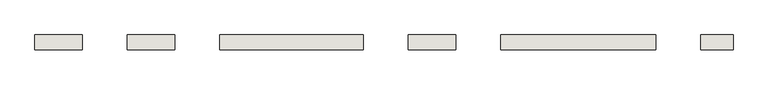
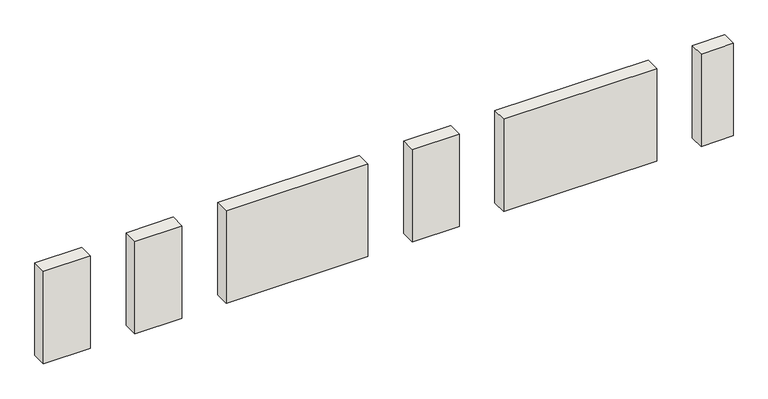
"""IFC4 building model written with IfcOpenShell, lengths in millimetres: wall geometry, 0_3d."""

import ifcopenshell
import ifcopenshell.guid

model = None  # the IFC model being written
_history = None  # IfcOwnerHistory: only IFC2X3 demands one
_inside = {}  # id of a spatial element -> (the spatial element, [elements in it])
_under = {}  # id of a project, library or spatial element -> (it, [spatial elements below it])
_declared = {}  # id of a project -> (the project, [libraries it declares])
_typed = {}  # id of a type object -> (the type object, [elements of that type])
_made_of = {}  # id of a material, layer set ... -> (it, [elements and type objects made of it])


def new_model(schema):
    """Start an empty IFC model of exactly this schema.

    Asked for "IFC4X3", IfcOpenShell would pick the latest addendum, in which some entities
    have other attributes; the version numbers below select the first issue.
    IFC2X3 requires an IfcOwnerHistory on every rooted entity: one is made here for all.
    """
    global model, _history
    if schema == "IFC4X3":
        model = ifcopenshell.file(schema_version=(4, 3, 0, 0))
    else:
        model = ifcopenshell.file(schema=schema)
    _inside.clear()
    _under.clear()
    _declared.clear()
    _typed.clear()
    _made_of.clear()
    _history = None
    if model.schema == "IFC2X3":
        org = make("IfcOrganization", Name="unknown")
        user = make(
            "IfcPersonAndOrganization",
            ThePerson=make("IfcPerson", FamilyName="unknown"),
            TheOrganization=org,
        )
        app = make(
            "IfcApplication",
            ApplicationDeveloper=org,
            Version="unknown",
            ApplicationFullName="unknown",
            ApplicationIdentifier="unknown",
        )
        _history = make(
            "IfcOwnerHistory",
            OwningUser=user,
            OwningApplication=app,
            ChangeAction="ADDED",
            CreationDate=0,
        )
    return model


def make(cls, **values):
    """One entity of the class cls with the attributes given. An attribute that is None is left unset."""
    return model.create_entity(
        cls, **{name: value for name, value in values.items() if value is not None}
    )


def rooted(cls, **values):
    """An entity with a GlobalId (a new one), such as an element, a storey or a relation."""
    return make(cls, GlobalId=ifcopenshell.guid.new(), OwnerHistory=_history, **values)


def si_unit(unit_type, name, prefix=None):
    """IfcSIUnit, for example si_unit("LENGTHUNIT", "METRE", prefix="MILLI")."""
    return make("IfcSIUnit", UnitType=unit_type, Prefix=prefix, Name=name)


def assignment(units):
    """IfcUnitAssignment: the units of a project."""
    return None if units is None else make("IfcUnitAssignment", Units=units)


def point(xyz):
    """IfcCartesianPoint."""
    return None if xyz is None else make("IfcCartesianPoint", Coordinates=xyz)


def direction(xyz):
    """IfcDirection."""
    return None if xyz is None else make("IfcDirection", DirectionRatios=xyz)


def frame(location, z_axis=None, x_axis=None):
    """IfcAxis2Placement3D, a coordinate frame: its origin and axes. An axis left out is left unset."""
    return make(
        "IfcAxis2Placement3D",
        Location=point(location),
        Axis=direction(z_axis),
        RefDirection=direction(x_axis),
    )


def origin():
    """The frame at (0, 0, 0) with its axes left unset."""
    return frame((0.0, 0.0, 0.0))


def origin_with_axes():
    """The frame at (0, 0, 0) with the z axis (0, 0, 1) and the x axis (1, 0, 0) written out."""
    return frame((0.0, 0.0, 0.0), z_axis=(0.0, 0.0, 1.0), x_axis=(1.0, 0.0, 0.0))


def place(relative_to, where):
    """IfcLocalPlacement: puts the frame where relative to a parent placement (None: the world)."""
    return make(
        "IfcLocalPlacement", PlacementRelTo=relative_to, RelativePlacement=where
    )


def context(
    kind, dimensions, precision=None, world=None, true_north=None, identifier=None
):
    """IfcGeometricRepresentationContext, for example the 3D "Model" context."""
    return make(
        "IfcGeometricRepresentationContext",
        ContextIdentifier=identifier,
        ContextType=kind,
        CoordinateSpaceDimension=dimensions,
        Precision=precision,
        WorldCoordinateSystem=world,
        TrueNorth=true_north,
    )


def project(units=None, contexts=None):
    """IfcProject with its units and contexts."""
    return rooted(
        "IfcProject",
        Name="project",
        RepresentationContexts=contexts,
        UnitsInContext=assignment(units),
    )


def spatial(cls, under=None, at=None, **own):
    """A site, building, storey or space (cls), placed at a placement, below another one or the project."""
    s = rooted(cls, ObjectPlacement=at, **own)
    if under is not None:
        _under.setdefault(under.id(), (under, []))[1].append(s)
    return s


def polyline(points):
    """IfcPolyline through the points."""
    return make("IfcPolyline", Points=[point(p) for p in points])


def outline(outer, holes=None, kind="AREA"):
    """IfcArbitraryClosedProfileDef: a profile drawn as a closed curve; with holes, ...WithVoids."""
    if holes is None:
        return make("IfcArbitraryClosedProfileDef", ProfileType=kind, OuterCurve=outer)
    return make(
        "IfcArbitraryProfileDefWithVoids",
        ProfileType=kind,
        OuterCurve=outer,
        InnerCurves=holes,
    )


def extrude(swept, where, along, depth):
    """IfcExtrudedAreaSolid: the profile swept, set in the frame where, extruded along a direction by depth."""
    return make(
        "IfcExtrudedAreaSolid",
        SweptArea=swept,
        Position=where,
        ExtrudedDirection=direction(along),
        Depth=depth,
    )


def shape(context_of_items, identifier, shape_type, items):
    """IfcShapeRepresentation: the items that make up one representation, for example the "Body"."""
    return make(
        "IfcShapeRepresentation",
        ContextOfItems=context_of_items,
        RepresentationIdentifier=identifier,
        RepresentationType=shape_type,
        Items=items,
    )


def source(mapping_origin, context_of_items, identifier, shape_type, items):
    """IfcRepresentationMap: a shape defined once, which mapped items show again and again."""
    return make(
        "IfcRepresentationMap",
        MappingOrigin=mapping_origin,
        MappedRepresentation=shape(context_of_items, identifier, shape_type, items),
    )


def transform(
    local_origin,
    x_axis=None,
    y_axis=None,
    z_axis=None,
    scale=None,
    scale2=None,
    scale3=None,
    uniform=True,
):
    """IfcCartesianTransformationOperator3D, or its non-uniform kind. x_axis, y_axis, z_axis: its Axis1, 2, 3."""
    if uniform:
        return make(
            "IfcCartesianTransformationOperator3D",
            Axis1=direction(x_axis),
            Axis2=direction(y_axis),
            LocalOrigin=point(local_origin),
            Scale=scale,
            Axis3=direction(z_axis),
        )
    return make(
        "IfcCartesianTransformationOperator3DnonUniform",
        Axis1=direction(x_axis),
        Axis2=direction(y_axis),
        LocalOrigin=point(local_origin),
        Scale=scale,
        Axis3=direction(z_axis),
        Scale2=scale2,
        Scale3=scale3,
    )


def mapped(mapping_source, mapping_target):
    """IfcMappedItem: shows the shape of a source again, moved by a transform."""
    return make(
        "IfcMappedItem", MappingSource=mapping_source, MappingTarget=mapping_target
    )


def made_of(thing, what):
    """Note that an element or type object is made of a material, layer set ...; save() writes the relation."""
    if what is not None:
        _made_of.setdefault(what.id(), (what, []))[1].append(thing)
    return thing


def element(
    cls,
    number,
    at=None,
    inside=None,
    cuts=None,
    type_object=None,
    material=None,
    context=None,
    identifier="Body",
    shape_type=None,
    held_by="IfcProductDefinitionShape",
    body=None,
    shapes=None,
    **own,
):
    """One element of the class cls, such as IfcWall. Its Tag is "e" and its number.

    at: its placement. inside: the storey or other place that contains it. cuts: it is an
    opening in that element (IfcRelVoidsElement). A single representation is given by context,
    identifier, shape_type and body (its items); several are given by shapes. held_by: the class
    of the entity that holds the representations. save() writes the other relations.
    """
    e = rooted(cls, Tag="e%d" % number, ObjectPlacement=at, **own)
    if body is not None:
        shapes = [shape(context, identifier, shape_type, body)]
    if shapes is not None:
        e.Representation = make(held_by, Representations=shapes)
    if inside is not None:
        _inside.setdefault(inside.id(), (inside, []))[1].append(e)
    if cuts is not None:
        rooted(
            "IfcRelVoidsElement", RelatingBuildingElement=cuts, RelatedOpeningElement=e
        )
    if type_object is not None:
        _typed.setdefault(type_object.id(), (type_object, []))[1].append(e)
    return made_of(e, material)


def aggregate(whole, parts):
    """IfcRelAggregates: a whole, such as a stair, and the parts it consists of."""
    return rooted("IfcRelAggregates", RelatingObject=whole, RelatedObjects=parts)


def save(model, path):
    """Write the relations noted so far, then the file.

    IfcRelAggregates (storeys below a building ...), IfcRelContainedInSpatialStructure (elements
    in a storey), IfcRelDefinesByType, IfcRelAssociatesMaterial and IfcRelDeclares: one each for
    every whole, place, type object, material and project.
    """
    for whole, parts in _under.values():
        aggregate(whole, parts)
    for where, things in _inside.values():
        rooted(
            "IfcRelContainedInSpatialStructure",
            RelatedElements=things,
            RelatingStructure=where,
        )
    for kind, things in _typed.values():
        rooted("IfcRelDefinesByType", RelatedObjects=things, RelatingType=kind)
    for what, things in _made_of.values():
        rooted("IfcRelAssociatesMaterial", RelatedObjects=things, RelatingMaterial=what)
    for by, libraries in _declared.values():
        rooted("IfcRelDeclares", RelatingContext=by, RelatedDefinitions=libraries)
    model.write(path)


def wall_31735f31(model_context):
    return source(origin(), model_context, "Body", "SweptSolid", [
        extrude(outline(polyline([(1200.0, 380.0), (1200.0, 0.0), (0.0, 0.0), (0.0, 380.0), (1200.0, 380.0)])), origin_with_axes(), (0.0, 0.0, 1.0), 2500.0),
        extrude(outline(polyline([(2335.0, 0.0), (2335.0, 380.0), (3533.0664986, 380.0), (3533.0664986, 0.0), (2335.0, 0.0)])), origin_with_axes(), (0.0, 0.0, 1.0), 2500.0),
        extrude(outline(polyline([(8287.897415, 380.0), (8287.897415, 0.0), (4668.0664986, 0.0), (4668.0664986, 380.0), (8287.897415, 380.0)])), origin_with_axes(), (0.0, 0.0, 1.0), 2500.0),
        extrude(outline(polyline([(9422.897415, 0.0), (9422.897415, 380.0), (10622.5, 380.0), (10622.5, 0.0), (9422.897415, 0.0)])), origin_with_axes(), (0.0, 0.0, 1.0), 2500.0),
        extrude(outline(polyline([(15668.2593169, 380.0), (15668.2593169, 0.0), (11757.5, 0.0), (11757.5, 380.0), (15668.2593169, 380.0)])), origin_with_axes(), (0.0, 0.0, 1.0), 2500.0),
        extrude(outline(polyline([(16803.2593169, 0.0), (16803.2593169, 380.0), (17622.8619019, 380.0), (17622.8619019, 0.0), (16803.2593169, 0.0)])), origin_with_axes(), (0.0, 0.0, 1.0), 2500.0),
    ])


if __name__ == "__main__":
    model = new_model("IFC4")
    model_context = context("Model", 3, world=origin())
    ifc_project = project(units=[si_unit("LENGTHUNIT", "METRE", prefix="MILLI")], contexts=[model_context])
    site = spatial("IfcSite", under=ifc_project)
    building = spatial("IfcBuilding", under=site)
    placement = place(None, origin())
    wall_shape = wall_31735f31(model_context)
    element("IfcWall", 1, ObjectType="0_3d", at=placement, inside=building, context=model_context, shape_type="MappedRepresentation", body=[
        mapped(wall_shape, transform((0.0, 0.0, 0.0), x_axis=(1.0, 0.0, 0.0), y_axis=(0.0, 1.0, 0.0), z_axis=(0.0, 0.0, 1.0))),
    ])
    save(model, "model.ifc")

# Revit data of these elements
# Element 1 (IfcWall, "0_3d")
#   Materials on its faces: "holzschalung"
# Materials
#   "holzschalung": class "Unassigned", colour RGB 128 128 128, transparency 0
